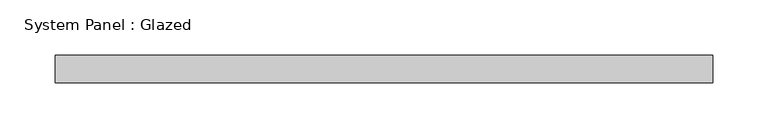
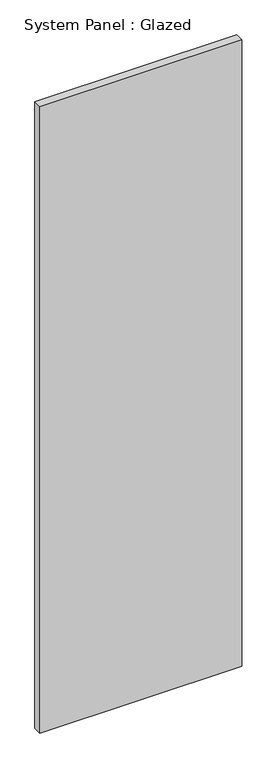
"""IFC4 building model written with IfcOpenShell, lengths in millimetres: plate geometry, System Panel : Glazed."""

from ifc_helpers import new_model, si_unit, origin, origin_with_axes, place, context, project, spatial, polyline, outline, extrude, source, transform, mapped, element, save


def system_panel_glazed_84d9e71a(model_context):
    return source(origin(), model_context, "Body", "SweptSolid", [
        extrude(outline(polyline([(297.5, 24.5), (-297.5, 24.5), (-297.5, 49.5), (297.5, 49.5), (297.5, 24.5)])), origin_with_axes(), (0.0, 0.0, 1.0), 1950.0),
    ])


if __name__ == "__main__":
    model = new_model("IFC4")
    model_context = context("Model", 3, world=origin())
    ifc_project = project(units=[si_unit("LENGTHUNIT", "METRE", prefix="MILLI")], contexts=[model_context])
    site = spatial("IfcSite", under=ifc_project)
    building = spatial("IfcBuilding", under=site)
    placement = place(None, origin())
    system_panel_glazed_shape = system_panel_glazed_84d9e71a(model_context)
    element("IfcPlate", 1, ObjectType="System Panel : Glazed", at=placement, inside=building, context=model_context, shape_type="MappedRepresentation", body=[
        mapped(system_panel_glazed_shape, transform((0.0, 0.0, 0.0), x_axis=(1.0, 0.0, 0.0), y_axis=(0.0, 1.0, 0.0), z_axis=(0.0, 0.0, 1.0))),
    ])
    save(model, "model.ifc")

# Revit data of these elements
# Element 1 (IfcPlate, "System Panel : Glazed")
#   Materials on its faces: "Glass"
# Materials
#   "Glass": class "Glass", colour RGB 0 128 192, transparency 0.9
